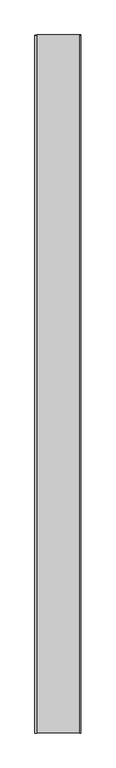
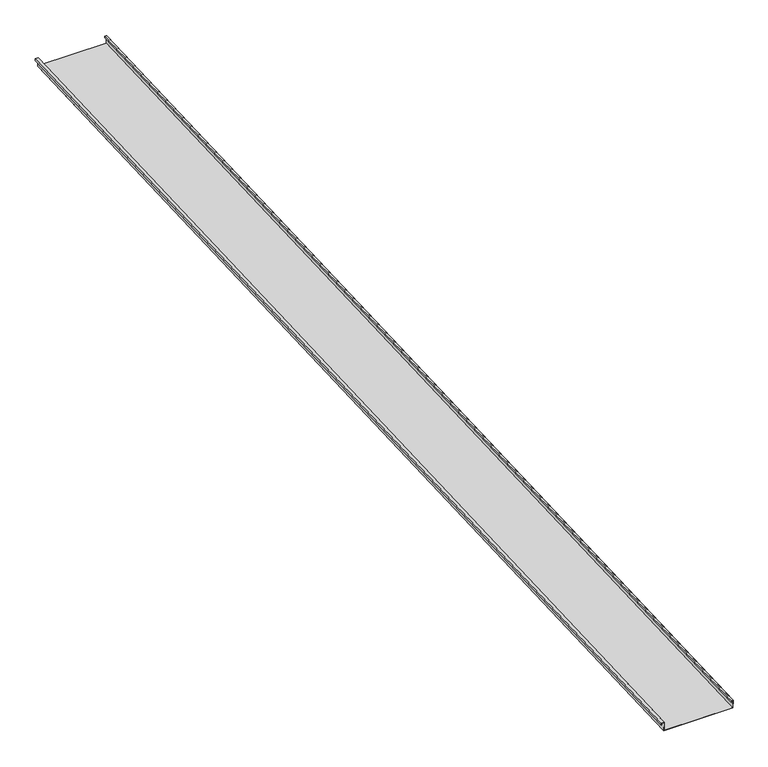
"""IFC4 building model written with IfcOpenShell, lengths in millimetres: proxy geometry, Generic Models 2:Generic Models 2:310765:Generic Models 2:310765 : Generic Models 2:Generic Models 2:310765:131 : Generic Models 2:Generic Models 2:310765:Generic Models 2:310765 : Generic Models 2:Generic Models 2:310765:300385."""

import ifcopenshell
import ifcopenshell.guid

model = None  # the IFC model being written
_history = None  # IfcOwnerHistory: only IFC2X3 demands one
_inside = {}  # id of a spatial element -> (the spatial element, [elements in it])
_under = {}  # id of a project, library or spatial element -> (it, [spatial elements below it])
_declared = {}  # id of a project -> (the project, [libraries it declares])
_typed = {}  # id of a type object -> (the type object, [elements of that type])
_made_of = {}  # id of a material, layer set ... -> (it, [elements and type objects made of it])


def new_model(schema):
    """Start an empty IFC model of exactly this schema.

    Asked for "IFC4X3", IfcOpenShell would pick the latest addendum, in which some entities
    have other attributes; the version numbers below select the first issue.
    IFC2X3 requires an IfcOwnerHistory on every rooted entity: one is made here for all.
    """
    global model, _history
    if schema == "IFC4X3":
        model = ifcopenshell.file(schema_version=(4, 3, 0, 0))
    else:
        model = ifcopenshell.file(schema=schema)
    _inside.clear()
    _under.clear()
    _declared.clear()
    _typed.clear()
    _made_of.clear()
    _history = None
    if model.schema == "IFC2X3":
        org = make("IfcOrganization", Name="unknown")
        user = make(
            "IfcPersonAndOrganization",
            ThePerson=make("IfcPerson", FamilyName="unknown"),
            TheOrganization=org,
        )
        app = make(
            "IfcApplication",
            ApplicationDeveloper=org,
            Version="unknown",
            ApplicationFullName="unknown",
            ApplicationIdentifier="unknown",
        )
        _history = make(
            "IfcOwnerHistory",
            OwningUser=user,
            OwningApplication=app,
            ChangeAction="ADDED",
            CreationDate=0,
        )
    return model


def make(cls, **values):
    """One entity of the class cls with the attributes given. An attribute that is None is left unset."""
    return model.create_entity(
        cls, **{name: value for name, value in values.items() if value is not None}
    )


def rooted(cls, **values):
    """An entity with a GlobalId (a new one), such as an element, a storey or a relation."""
    return make(cls, GlobalId=ifcopenshell.guid.new(), OwnerHistory=_history, **values)


def si_unit(unit_type, name, prefix=None):
    """IfcSIUnit, for example si_unit("LENGTHUNIT", "METRE", prefix="MILLI")."""
    return make("IfcSIUnit", UnitType=unit_type, Prefix=prefix, Name=name)


def assignment(units):
    """IfcUnitAssignment: the units of a project."""
    return None if units is None else make("IfcUnitAssignment", Units=units)


def point(xyz):
    """IfcCartesianPoint."""
    return None if xyz is None else make("IfcCartesianPoint", Coordinates=xyz)


def direction(xyz):
    """IfcDirection."""
    return None if xyz is None else make("IfcDirection", DirectionRatios=xyz)


def frame(location, z_axis=None, x_axis=None):
    """IfcAxis2Placement3D, a coordinate frame: its origin and axes. An axis left out is left unset."""
    return make(
        "IfcAxis2Placement3D",
        Location=point(location),
        Axis=direction(z_axis),
        RefDirection=direction(x_axis),
    )


def origin():
    """The frame at (0, 0, 0) with its axes left unset."""
    return frame((0.0, 0.0, 0.0))


def place(relative_to, where):
    """IfcLocalPlacement: puts the frame where relative to a parent placement (None: the world)."""
    return make(
        "IfcLocalPlacement", PlacementRelTo=relative_to, RelativePlacement=where
    )


def context(
    kind, dimensions, precision=None, world=None, true_north=None, identifier=None
):
    """IfcGeometricRepresentationContext, for example the 3D "Model" context."""
    return make(
        "IfcGeometricRepresentationContext",
        ContextIdentifier=identifier,
        ContextType=kind,
        CoordinateSpaceDimension=dimensions,
        Precision=precision,
        WorldCoordinateSystem=world,
        TrueNorth=true_north,
    )


def project(units=None, contexts=None):
    """IfcProject with its units and contexts."""
    return rooted(
        "IfcProject",
        Name="project",
        RepresentationContexts=contexts,
        UnitsInContext=assignment(units),
    )


def spatial(cls, under=None, at=None, **own):
    """A site, building, storey or space (cls), placed at a placement, below another one or the project."""
    s = rooted(cls, ObjectPlacement=at, **own)
    if under is not None:
        _under.setdefault(under.id(), (under, []))[1].append(s)
    return s


def polyline(points):
    """IfcPolyline through the points."""
    return make("IfcPolyline", Points=[point(p) for p in points])


def outline(outer, holes=None, kind="AREA"):
    """IfcArbitraryClosedProfileDef: a profile drawn as a closed curve; with holes, ...WithVoids."""
    if holes is None:
        return make("IfcArbitraryClosedProfileDef", ProfileType=kind, OuterCurve=outer)
    return make(
        "IfcArbitraryProfileDefWithVoids",
        ProfileType=kind,
        OuterCurve=outer,
        InnerCurves=holes,
    )


def extrude(swept, where, along, depth):
    """IfcExtrudedAreaSolid: the profile swept, set in the frame where, extruded along a direction by depth."""
    return make(
        "IfcExtrudedAreaSolid",
        SweptArea=swept,
        Position=where,
        ExtrudedDirection=direction(along),
        Depth=depth,
    )


def shape(context_of_items, identifier, shape_type, items):
    """IfcShapeRepresentation: the items that make up one representation, for example the "Body"."""
    return make(
        "IfcShapeRepresentation",
        ContextOfItems=context_of_items,
        RepresentationIdentifier=identifier,
        RepresentationType=shape_type,
        Items=items,
    )


def source(mapping_origin, context_of_items, identifier, shape_type, items):
    """IfcRepresentationMap: a shape defined once, which mapped items show again and again."""
    return make(
        "IfcRepresentationMap",
        MappingOrigin=mapping_origin,
        MappedRepresentation=shape(context_of_items, identifier, shape_type, items),
    )


def transform(
    local_origin,
    x_axis=None,
    y_axis=None,
    z_axis=None,
    scale=None,
    scale2=None,
    scale3=None,
    uniform=True,
):
    """IfcCartesianTransformationOperator3D, or its non-uniform kind. x_axis, y_axis, z_axis: its Axis1, 2, 3."""
    if uniform:
        return make(
            "IfcCartesianTransformationOperator3D",
            Axis1=direction(x_axis),
            Axis2=direction(y_axis),
            LocalOrigin=point(local_origin),
            Scale=scale,
            Axis3=direction(z_axis),
        )
    return make(
        "IfcCartesianTransformationOperator3DnonUniform",
        Axis1=direction(x_axis),
        Axis2=direction(y_axis),
        LocalOrigin=point(local_origin),
        Scale=scale,
        Axis3=direction(z_axis),
        Scale2=scale2,
        Scale3=scale3,
    )


def mapped(mapping_source, mapping_target):
    """IfcMappedItem: shows the shape of a source again, moved by a transform."""
    return make(
        "IfcMappedItem", MappingSource=mapping_source, MappingTarget=mapping_target
    )


def made_of(thing, what):
    """Note that an element or type object is made of a material, layer set ...; save() writes the relation."""
    if what is not None:
        _made_of.setdefault(what.id(), (what, []))[1].append(thing)
    return thing


def element(
    cls,
    number,
    at=None,
    inside=None,
    cuts=None,
    type_object=None,
    material=None,
    context=None,
    identifier="Body",
    shape_type=None,
    held_by="IfcProductDefinitionShape",
    body=None,
    shapes=None,
    **own,
):
    """One element of the class cls, such as IfcWall. Its Tag is "e" and its number.

    at: its placement. inside: the storey or other place that contains it. cuts: it is an
    opening in that element (IfcRelVoidsElement). A single representation is given by context,
    identifier, shape_type and body (its items); several are given by shapes. held_by: the class
    of the entity that holds the representations. save() writes the other relations.
    """
    e = rooted(cls, Tag="e%d" % number, ObjectPlacement=at, **own)
    if body is not None:
        shapes = [shape(context, identifier, shape_type, body)]
    if shapes is not None:
        e.Representation = make(held_by, Representations=shapes)
    if inside is not None:
        _inside.setdefault(inside.id(), (inside, []))[1].append(e)
    if cuts is not None:
        rooted(
            "IfcRelVoidsElement", RelatingBuildingElement=cuts, RelatedOpeningElement=e
        )
    if type_object is not None:
        _typed.setdefault(type_object.id(), (type_object, []))[1].append(e)
    return made_of(e, material)


def aggregate(whole, parts):
    """IfcRelAggregates: a whole, such as a stair, and the parts it consists of."""
    return rooted("IfcRelAggregates", RelatingObject=whole, RelatedObjects=parts)


def save(model, path):
    """Write the relations noted so far, then the file.

    IfcRelAggregates (storeys below a building ...), IfcRelContainedInSpatialStructure (elements
    in a storey), IfcRelDefinesByType, IfcRelAssociatesMaterial and IfcRelDeclares: one each for
    every whole, place, type object, material and project.
    """
    for whole, parts in _under.values():
        aggregate(whole, parts)
    for where, things in _inside.values():
        rooted(
            "IfcRelContainedInSpatialStructure",
            RelatedElements=things,
            RelatingStructure=where,
        )
    for kind, things in _typed.values():
        rooted("IfcRelDefinesByType", RelatedObjects=things, RelatingType=kind)
    for what, things in _made_of.values():
        rooted("IfcRelAssociatesMaterial", RelatedObjects=things, RelatingMaterial=what)
    for by, libraries in _declared.values():
        rooted("IfcRelDeclares", RelatingContext=by, RelatedDefinitions=libraries)
    model.write(path)


def generic_models_50fb350e(model_context):
    return source(origin(), model_context, "Body", "SweptSolid", [
        extrude(outline(polyline([(1.5875, 0.0), (1.5875, 50.8), (407.9875, 50.8), (407.9875, 1.5875), (396.875, 1.5875), (396.875, 11.1125), (398.4625, 11.1125), (398.4625, 3.175), (406.4, 3.175), (406.4, 49.2125), (3.175, 49.2125), (3.175, -1.5874999), (-14.2875, -1.5874999), (-14.2875, 9.525), (-12.7, 9.525), (-12.7, 0.0), (1.5875, 0.0)])), frame((660941.4596405, -581354.4345603, 3902.6697972), z_axis=(0.0, 0.9991330730923568, 0.041630544712067834), x_axis=(1.0, 0.0, 0.0)), (0.0, 0.0, 1.0), 6400.8),
    ])


if __name__ == "__main__":
    model = new_model("IFC4")
    model_context = context("Model", 3, world=origin())
    ifc_project = project(units=[si_unit("LENGTHUNIT", "METRE", prefix="MILLI")], contexts=[model_context])
    site = spatial("IfcSite", under=ifc_project)
    building = spatial("IfcBuilding", under=site)
    placement = place(None, origin())
    generic_models_shape = generic_models_50fb350e(model_context)
    element("IfcBuildingElementProxy", 1, Name="Generic Models 2:Generic Models 2:310765:Generic Models 2:310765 : Generic Models 2:Generic Models 2:310765:131 : Generic Models 2:Generic Models 2:310765:Generic Models 2:310765 : Generic Models 2:Generic Models 2:310765:300385", ObjectType="Generic Models 2:Generic Models 2:310765:Generic Models 2:310765 : Generic Models 2:Generic Models 2:310765:131 : Generic Models 2:Generic Models 2:310765:Generic Models 2:310765 : Generic Models 2:Generic Models 2:310765:300385", at=placement, inside=building, context=model_context, shape_type="MappedRepresentation", body=[
        mapped(generic_models_shape, transform((0.0, 0.0, 0.0), x_axis=(1.0, 0.0, 0.0), y_axis=(0.0, 1.0, 0.0), z_axis=(0.0, 0.0, 1.0))),
    ])
    save(model, "model.ifc")

# Revit data of these elements
# Type "Generic Models 2:Generic Models 2:310765:Generic Models 2:310765 : Generic Models 2:Generic Models 2:310765:131 : Generic Models 2:Generic Models 2:310765:Generic Models 2:310765 : Generic Models 2:Generic Models 2:310765:300385"
#   NameOverride = "Generic Models 2:Generic Models 2:310765:Generic Models 2:310765 : Generic Models 2:Generic Models 2:310765:300385"
#   ObjectTypeOverride = "Generic Models 2:310765 : Generic Models 2:Generic Models 2:310765"
#   Reference = "Generic Models 2"
#   Tag = "300385"
# Element 1 (IfcBuildingElementProxy, "Generic Models 2:Generic Models 2:310765:Generic Models 2:310765 : Generic Models 2:Generic Models 2:310765:131 : Generic Models 2:Generic Models 2:310765:Generic Models 2:310765 : Generic Models 2:Generic Models 2:310765:300385")
#   Materials on its faces: "THERMAL BROKEN ALUMINUM STOREFRONT FOR POLYCARBONATE"
# Materials
#   "THERMAL BROKEN ALUMINUM STOREFRONT FOR POLYCARBONATE": class "Unassigned", colour RGB 244 244 244, transparency 0, Keynote = "M07611300.01", Cost = 0
